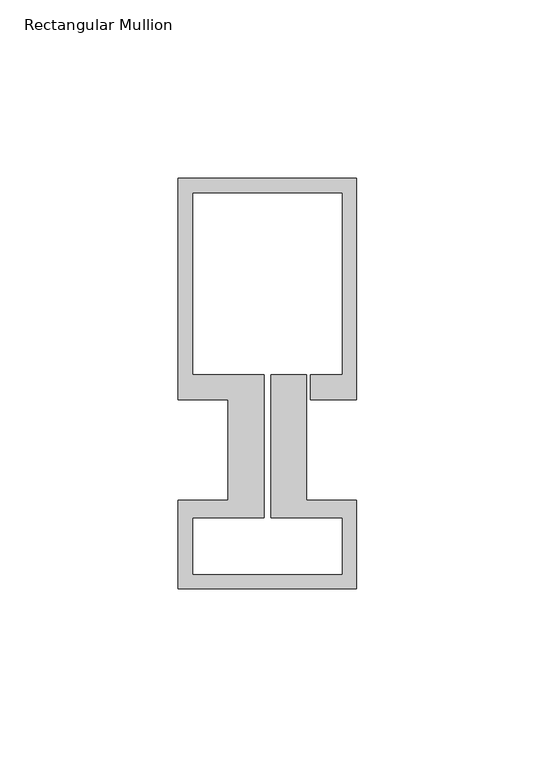
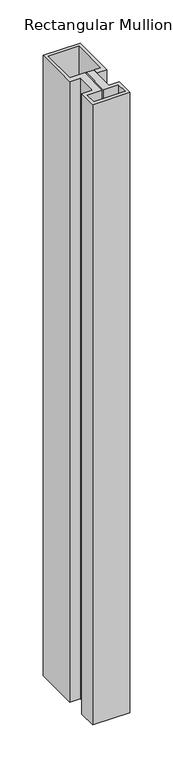
"""IFC4 building model written with IfcOpenShell, lengths in millimetres: member geometry, Rectangular Mullion : Schueco_FWS-50-HI_Tran_CovCap-20mm_Tran-55mm."""

import ifcopenshell
import ifcopenshell.guid

model = None  # the IFC model being written
_history = None  # IfcOwnerHistory: only IFC2X3 demands one
_inside = {}  # id of a spatial element -> (the spatial element, [elements in it])
_under = {}  # id of a project, library or spatial element -> (it, [spatial elements below it])
_declared = {}  # id of a project -> (the project, [libraries it declares])
_typed = {}  # id of a type object -> (the type object, [elements of that type])
_made_of = {}  # id of a material, layer set ... -> (it, [elements and type objects made of it])


def new_model(schema):
    """Start an empty IFC model of exactly this schema.

    Asked for "IFC4X3", IfcOpenShell would pick the latest addendum, in which some entities
    have other attributes; the version numbers below select the first issue.
    IFC2X3 requires an IfcOwnerHistory on every rooted entity: one is made here for all.
    """
    global model, _history
    if schema == "IFC4X3":
        model = ifcopenshell.file(schema_version=(4, 3, 0, 0))
    else:
        model = ifcopenshell.file(schema=schema)
    _inside.clear()
    _under.clear()
    _declared.clear()
    _typed.clear()
    _made_of.clear()
    _history = None
    if model.schema == "IFC2X3":
        org = make("IfcOrganization", Name="unknown")
        user = make(
            "IfcPersonAndOrganization",
            ThePerson=make("IfcPerson", FamilyName="unknown"),
            TheOrganization=org,
        )
        app = make(
            "IfcApplication",
            ApplicationDeveloper=org,
            Version="unknown",
            ApplicationFullName="unknown",
            ApplicationIdentifier="unknown",
        )
        _history = make(
            "IfcOwnerHistory",
            OwningUser=user,
            OwningApplication=app,
            ChangeAction="ADDED",
            CreationDate=0,
        )
    return model


def make(cls, **values):
    """One entity of the class cls with the attributes given. An attribute that is None is left unset."""
    return model.create_entity(
        cls, **{name: value for name, value in values.items() if value is not None}
    )


def rooted(cls, **values):
    """An entity with a GlobalId (a new one), such as an element, a storey or a relation."""
    return make(cls, GlobalId=ifcopenshell.guid.new(), OwnerHistory=_history, **values)


def si_unit(unit_type, name, prefix=None):
    """IfcSIUnit, for example si_unit("LENGTHUNIT", "METRE", prefix="MILLI")."""
    return make("IfcSIUnit", UnitType=unit_type, Prefix=prefix, Name=name)


def assignment(units):
    """IfcUnitAssignment: the units of a project."""
    return None if units is None else make("IfcUnitAssignment", Units=units)


def point(xyz):
    """IfcCartesianPoint."""
    return None if xyz is None else make("IfcCartesianPoint", Coordinates=xyz)


def direction(xyz):
    """IfcDirection."""
    return None if xyz is None else make("IfcDirection", DirectionRatios=xyz)


def frame(location, z_axis=None, x_axis=None):
    """IfcAxis2Placement3D, a coordinate frame: its origin and axes. An axis left out is left unset."""
    return make(
        "IfcAxis2Placement3D",
        Location=point(location),
        Axis=direction(z_axis),
        RefDirection=direction(x_axis),
    )


def origin():
    """The frame at (0, 0, 0) with its axes left unset."""
    return frame((0.0, 0.0, 0.0))


def place(relative_to, where):
    """IfcLocalPlacement: puts the frame where relative to a parent placement (None: the world)."""
    return make(
        "IfcLocalPlacement", PlacementRelTo=relative_to, RelativePlacement=where
    )


def context(
    kind, dimensions, precision=None, world=None, true_north=None, identifier=None
):
    """IfcGeometricRepresentationContext, for example the 3D "Model" context."""
    return make(
        "IfcGeometricRepresentationContext",
        ContextIdentifier=identifier,
        ContextType=kind,
        CoordinateSpaceDimension=dimensions,
        Precision=precision,
        WorldCoordinateSystem=world,
        TrueNorth=true_north,
    )


def project(units=None, contexts=None):
    """IfcProject with its units and contexts."""
    return rooted(
        "IfcProject",
        Name="project",
        RepresentationContexts=contexts,
        UnitsInContext=assignment(units),
    )


def spatial(cls, under=None, at=None, **own):
    """A site, building, storey or space (cls), placed at a placement, below another one or the project."""
    s = rooted(cls, ObjectPlacement=at, **own)
    if under is not None:
        _under.setdefault(under.id(), (under, []))[1].append(s)
    return s


def polyline(points):
    """IfcPolyline through the points."""
    return make("IfcPolyline", Points=[point(p) for p in points])


def outline(outer, holes=None, kind="AREA"):
    """IfcArbitraryClosedProfileDef: a profile drawn as a closed curve; with holes, ...WithVoids."""
    if holes is None:
        return make("IfcArbitraryClosedProfileDef", ProfileType=kind, OuterCurve=outer)
    return make(
        "IfcArbitraryProfileDefWithVoids",
        ProfileType=kind,
        OuterCurve=outer,
        InnerCurves=holes,
    )


def extrude(swept, where, along, depth):
    """IfcExtrudedAreaSolid: the profile swept, set in the frame where, extruded along a direction by depth."""
    return make(
        "IfcExtrudedAreaSolid",
        SweptArea=swept,
        Position=where,
        ExtrudedDirection=direction(along),
        Depth=depth,
    )


def shape(context_of_items, identifier, shape_type, items):
    """IfcShapeRepresentation: the items that make up one representation, for example the "Body"."""
    return make(
        "IfcShapeRepresentation",
        ContextOfItems=context_of_items,
        RepresentationIdentifier=identifier,
        RepresentationType=shape_type,
        Items=items,
    )


def source(mapping_origin, context_of_items, identifier, shape_type, items):
    """IfcRepresentationMap: a shape defined once, which mapped items show again and again."""
    return make(
        "IfcRepresentationMap",
        MappingOrigin=mapping_origin,
        MappedRepresentation=shape(context_of_items, identifier, shape_type, items),
    )


def transform(
    local_origin,
    x_axis=None,
    y_axis=None,
    z_axis=None,
    scale=None,
    scale2=None,
    scale3=None,
    uniform=True,
):
    """IfcCartesianTransformationOperator3D, or its non-uniform kind. x_axis, y_axis, z_axis: its Axis1, 2, 3."""
    if uniform:
        return make(
            "IfcCartesianTransformationOperator3D",
            Axis1=direction(x_axis),
            Axis2=direction(y_axis),
            LocalOrigin=point(local_origin),
            Scale=scale,
            Axis3=direction(z_axis),
        )
    return make(
        "IfcCartesianTransformationOperator3DnonUniform",
        Axis1=direction(x_axis),
        Axis2=direction(y_axis),
        LocalOrigin=point(local_origin),
        Scale=scale,
        Axis3=direction(z_axis),
        Scale2=scale2,
        Scale3=scale3,
    )


def mapped(mapping_source, mapping_target):
    """IfcMappedItem: shows the shape of a source again, moved by a transform."""
    return make(
        "IfcMappedItem", MappingSource=mapping_source, MappingTarget=mapping_target
    )


def made_of(thing, what):
    """Note that an element or type object is made of a material, layer set ...; save() writes the relation."""
    if what is not None:
        _made_of.setdefault(what.id(), (what, []))[1].append(thing)
    return thing


def element(
    cls,
    number,
    at=None,
    inside=None,
    cuts=None,
    type_object=None,
    material=None,
    context=None,
    identifier="Body",
    shape_type=None,
    held_by="IfcProductDefinitionShape",
    body=None,
    shapes=None,
    **own,
):
    """One element of the class cls, such as IfcWall. Its Tag is "e" and its number.

    at: its placement. inside: the storey or other place that contains it. cuts: it is an
    opening in that element (IfcRelVoidsElement). A single representation is given by context,
    identifier, shape_type and body (its items); several are given by shapes. held_by: the class
    of the entity that holds the representations. save() writes the other relations.
    """
    e = rooted(cls, Tag="e%d" % number, ObjectPlacement=at, **own)
    if body is not None:
        shapes = [shape(context, identifier, shape_type, body)]
    if shapes is not None:
        e.Representation = make(held_by, Representations=shapes)
    if inside is not None:
        _inside.setdefault(inside.id(), (inside, []))[1].append(e)
    if cuts is not None:
        rooted(
            "IfcRelVoidsElement", RelatingBuildingElement=cuts, RelatedOpeningElement=e
        )
    if type_object is not None:
        _typed.setdefault(type_object.id(), (type_object, []))[1].append(e)
    return made_of(e, material)


def aggregate(whole, parts):
    """IfcRelAggregates: a whole, such as a stair, and the parts it consists of."""
    return rooted("IfcRelAggregates", RelatingObject=whole, RelatedObjects=parts)


def save(model, path):
    """Write the relations noted so far, then the file.

    IfcRelAggregates (storeys below a building ...), IfcRelContainedInSpatialStructure (elements
    in a storey), IfcRelDefinesByType, IfcRelAssociatesMaterial and IfcRelDeclares: one each for
    every whole, place, type object, material and project.
    """
    for whole, parts in _under.values():
        aggregate(whole, parts)
    for where, things in _inside.values():
        rooted(
            "IfcRelContainedInSpatialStructure",
            RelatedElements=things,
            RelatingStructure=where,
        )
    for kind, things in _typed.values():
        rooted("IfcRelDefinesByType", RelatedObjects=things, RelatingType=kind)
    for what, things in _made_of.values():
        rooted("IfcRelAssociatesMaterial", RelatedObjects=things, RelatingMaterial=what)
    for by, libraries in _declared.values():
        rooted("IfcRelDeclares", RelatingContext=by, RelatedDefinitions=libraries)
    model.write(path)


def rectangular_mullion_66657b2f(model_context):
    return source(origin(), model_context, "Body", "SweptSolid", [
        extrude(outline(polyline([(-50.0, 90.0), (0.0, 90.0), (0.0, 28.0), (-13.0, 28.0), (-13.0, 35.0), (-4.0, 35.0), (-4.0, 86.0), (-46.0, 86.0), (-46.0, 35.0), (-26.0, 35.0), (-26.0, -5.0), (-46.0, -5.0), (-46.0, -21.0), (-4.0, -21.0), (-4.0, -5.0), (-24.0, -5.0), (-24.0, 35.0), (-14.0, 35.0), (-14.0, -0.1), (0.0, -0.1), (0.0, -25.0), (-50.0, -25.0), (-50.0, -0.1), (-36.0, -0.1), (-36.0, 28.0), (-50.0, 28.0), (-50.0, 90.0)])), frame((0.0, 0.0, -880.0), z_axis=(0.0, 0.0, 1.0), x_axis=(1.0, 0.0, 0.0)), (0.0, 0.0, 1.0), 880.0),
    ])


if __name__ == "__main__":
    model = new_model("IFC4")
    model_context = context("Model", 3, world=origin())
    ifc_project = project(units=[si_unit("LENGTHUNIT", "METRE", prefix="MILLI")], contexts=[model_context])
    site = spatial("IfcSite", under=ifc_project)
    building = spatial("IfcBuilding", under=site)
    placement = place(None, origin())
    rectangular_mullion_shape = rectangular_mullion_66657b2f(model_context)
    element("IfcMember", 1, ObjectType="Rectangular Mullion : Schueco_FWS-50-HI_Tran_CovCap-20mm_Tran-55mm", at=placement, inside=building, context=model_context, shape_type="MappedRepresentation", body=[
        mapped(rectangular_mullion_shape, transform((0.0, 0.0, 0.0), x_axis=(1.0, 0.0, 0.0), y_axis=(0.0, 1.0, 0.0), z_axis=(0.0, 0.0, 1.0))),
    ])
    save(model, "model.ifc")

# Revit data of these elements
# Type "Rectangular Mullion : Schueco_FWS-50-HI_Tran_CovCap-20mm_Tran-55mm"
#   Model = "FWS 50.HI"
#   Manufacturer = "Schueco International KG"
#   Type Comments = "Transom"
#   Schueco thermal insulation standard = "Highly thermally insulated"
#   Burglar resistance = "RC 3"
#   Thermal insulation = "to 0.90 W/(m²K)"
#   built-in parameter 1007322 = 0.377297 (stored number, unit not read)
#   built-in parameter 1007321 = 0.0360892 (stored number, unit not read)
#   built-in parameter 1007320 = 0.0360892 (stored number, unit not read)
# Element 1 (IfcMember, "Rectangular Mullion : Schueco_FWS-50-HI_Tran_CovCap-20mm_Tran-55mm")
#   Materials on its faces: "Alu"
# Materials
#   "Alu": class "Glas", colour RGB 140 140 140, transparency 0
